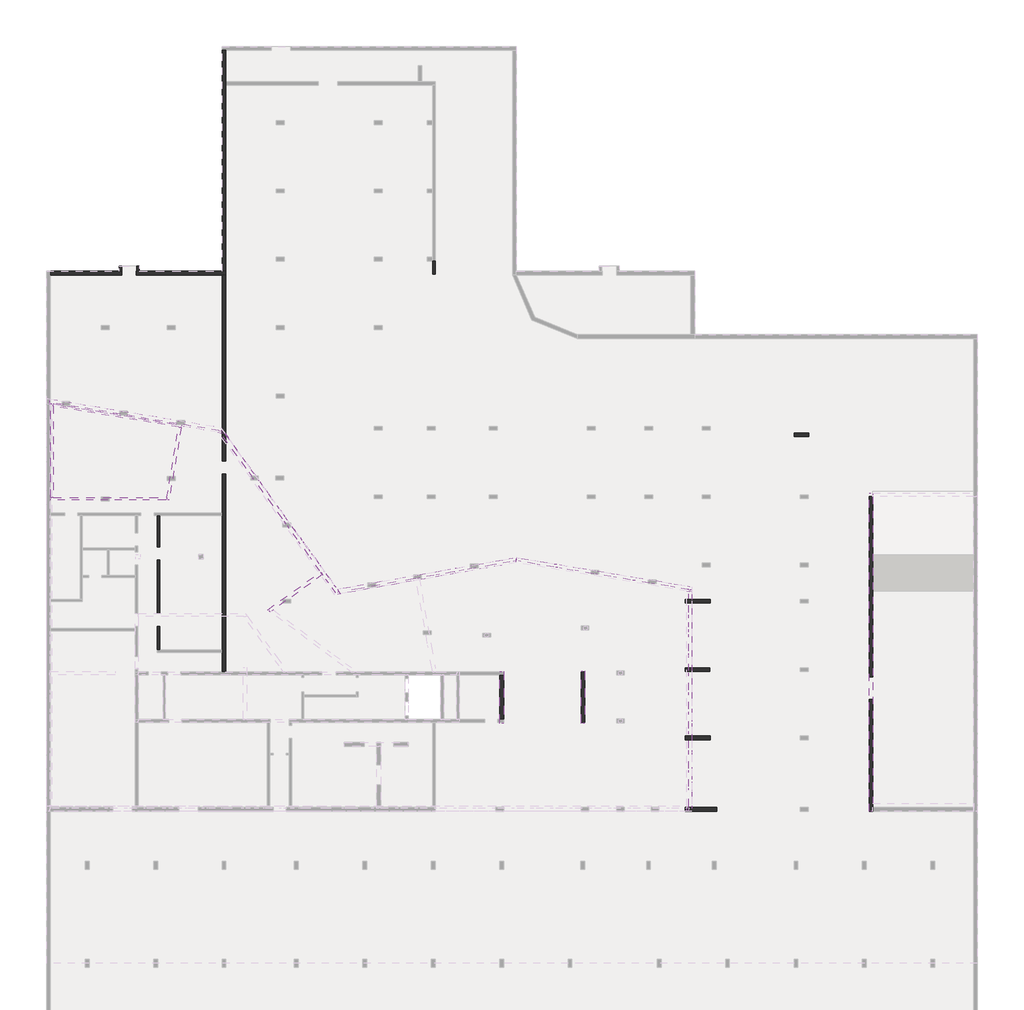
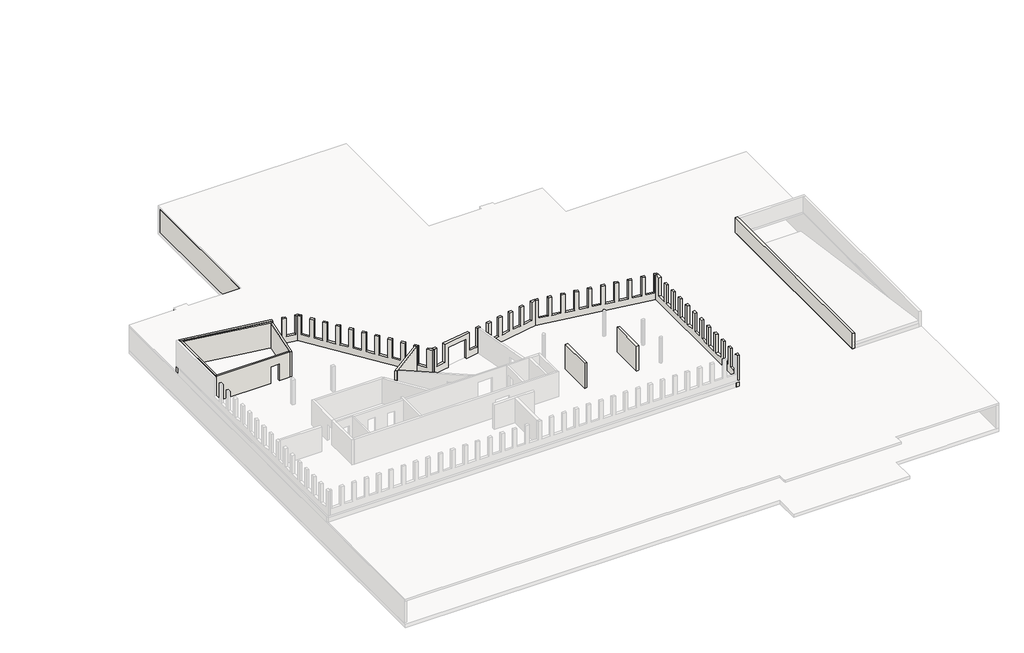
# One storey, part 3 of 4: 35 walls.
"""IFC4 building model written with IfcOpenShell, lengths in millimetres."""

from ifc_helpers import new_model, si_unit, point, frame, frame_2d, origin, place, context, project, spatial, polyline, circle_curve, trimmed, segment, composite_curve, outline, extrude, faceted_brep, element, save

model = new_model("IFC4")

# Units and contexts
model_context = context("Model", 3, world=origin())
ifc_project = project(units=[si_unit("LENGTHUNIT", "METRE", prefix="MILLI")], contexts=[model_context])

# Site, building, storey
site = spatial("IfcSite", under=ifc_project)
building = spatial("IfcBuilding", under=site)
storey = spatial("IfcBuildingStorey", under=building, Name="01_UG_OKFB_-4,20", Elevation=-4200.0)

# Walls
placement = place(None, origin())
element("IfcWall", 1, ObjectType="5dki Lochfassade 26cm C30/37", at=placement, inside=storey, context=model_context, shape_type="Brep", body=[
    faceted_brep([(13575.6085618, 29303.4331075, 3060.0), (13211.4553837, 29364.2425792, 3060.0), (12991.7792945, 29400.9260074, 3060.0), (12991.7792945, 29400.9260074, 710.0), (11926.5295409, 29578.8106961, 710.0), (11926.5295409, 29578.8106961, 3060.0), (11512.2657479, 29647.9880751, 3060.0), (11512.2657479, 29647.9880751, 710.0), (10447.0159943, 29825.8727639, 710.0), (10447.0159943, 29825.8727639, 3060.0), (130.0010047, 31548.6978518, 3060.0), (130.0010047, 31548.6978518, -150.0), (13211.4553837, 29364.2425792, -150.0), (13575.6085618, 29303.4331075, -150.0), (13034.6033862, 29657.3750221, 710.0), (13034.6033862, 29657.3750221, 3060.0), (13359.8955383, 29603.0549033, 3060.0), (13359.8955383, 29603.0549033, -150.0), (130.0010047, 31812.2980067, -150.0), (130.0010047, 31812.2980067, 3060.0), (10489.840086, 30082.3217786, 3060.0), (10489.840086, 30082.3217786, 710.0), (11555.0898396, 29904.4370898, 710.0), (11555.0898396, 29904.4370898, 3060.0), (11969.3536327, 29835.2597109, 3060.0), (11969.3536327, 29835.2597109, 710.0)], [[[0, 1, 2, 3, 4, 5, 6, 7, 8, 9, 10, 11, 12, 13]], [[14, 15, 16, 17, 18, 19, 20, 21, 22, 23, 24, 25]], [[13, 12, 11, 18, 17]], [[19, 10, 9, 20]], [[24, 23, 6, 5]], [[16, 15, 2, 1, 0]], [[11, 10, 19, 18]], [[0, 13, 17, 16]], [[8, 21, 20, 9]], [[22, 7, 6, 23]], [[21, 8, 7, 22]], [[5, 4, 25, 24]], [[3, 2, 15, 14]], [[4, 3, 14, 25]]]),
])
element("IfcWall", 2, ObjectType="5dki Lochfassade 26cm C30/37", at=placement, inside=storey, context=model_context, shape_type="Brep", body=[
    faceted_brep([(22268.004401, 16784.8468851, 3060.0), (21924.4906268, 17261.9817942, 3060.0), (21924.4906268, 17261.9817942, 710.0), (21293.4697845, 18138.4592307, 710.0), (21293.4697845, 18138.4592307, 3060.0), (21048.0727903, 18479.3115671, 3060.0), (21048.0727903, 18479.3115671, 710.0), (20417.0519481, 19355.7890035, 710.0), (20417.0519481, 19355.7890035, 3060.0), (20171.6549538, 19696.64134, 3060.0), (20171.6549538, 19696.64134, 710.0), (19540.6341116, 20573.1187764, 710.0), (19540.6341116, 20573.1187764, 3060.0), (19295.2371174, 20913.9711128, 3060.0), (19295.2371174, 20913.9711128, 710.0), (18664.2162751, 21790.4485493, 710.0), (18664.2162751, 21790.4485493, 3060.0), (18418.8192809, 22131.3008857, 3060.0), (18418.8192809, 22131.3008857, 710.0), (17787.7984387, 23007.7783222, 710.0), (17787.7984387, 23007.7783222, 3060.0), (17542.4014445, 23348.6306586, 3060.0), (17542.4014445, 23348.6306586, 710.0), (16911.3806022, 24225.1080951, 710.0), (16911.3806022, 24225.1080951, 3060.0), (16665.983608, 24565.9604315, 3060.0), (16665.983608, 24565.9604315, 710.0), (16034.9627658, 25442.4378679, 710.0), (16034.9627658, 25442.4378679, 3060.0), (15789.5657715, 25783.2902043, 3060.0), (15789.5657715, 25783.2902043, 710.0), (15158.5449293, 26659.7676408, 710.0), (15158.5449293, 26659.7676408, 3060.0), (14913.1479351, 27000.6199772, 3060.0), (14913.1479351, 27000.6199772, 710.0), (14282.1270928, 27877.0974137, 710.0), (14282.1270928, 27877.0974137, 3060.0), (14036.7300986, 28217.9497501, 3060.0), (14036.7300986, 28217.9497501, 710.0), (13405.7092564, 29094.4271866, 710.0), (13405.7092564, 29094.4271866, 3060.0), (13211.4553837, 29364.2425792, 3060.0), (13211.4553837, 29364.2425792, -150.0), (22268.004401, 16784.8468851, -150.0), (22135.4944541, 17413.8942192, 710.0), (22135.4944541, 17413.8942192, 3060.0), (22383.5041721, 17069.4128529, 3060.0), (22552.0750732, 16835.2706799, 3060.0), (22552.0750732, 16835.2706799, -150.0), (22383.5041721, 17069.4128529, -150.0), (13575.6085618, 29303.4331075, -150.0), (13575.6085618, 29303.4331075, 3060.0), (13616.7130837, 29246.3396115, 3060.0), (13616.7130837, 29246.3396115, 710.0), (14247.7339259, 28369.8621751, 710.0), (14247.7339259, 28369.8621751, 3060.0), (14493.1309201, 28029.0098387, 3060.0), (14493.1309201, 28029.0098387, 710.0), (15124.1517624, 27152.5324022, 710.0), (15124.1517624, 27152.5324022, 3060.0), (15369.5487566, 26811.6800658, 3060.0), (15369.5487566, 26811.6800658, 710.0), (16000.5695988, 25935.2026293, 710.0), (16000.5695988, 25935.2026293, 3060.0), (16245.966593, 25594.3502929, 3060.0), (16245.966593, 25594.3502929, 710.0), (16876.9874353, 24717.8728564, 710.0), (16876.9874353, 24717.8728564, 3060.0), (17122.3844295, 24377.02052, 3060.0), (17122.3844295, 24377.02052, 710.0), (17753.4052718, 23500.5430836, 710.0), (17753.4052718, 23500.5430836, 3060.0), (17998.802266, 23159.6907472, 3060.0), (17998.802266, 23159.6907472, 710.0), (18629.8231082, 22283.2133107, 710.0), (18629.8231082, 22283.2133107, 3060.0), (18875.2201024, 21942.3609743, 3060.0), (18875.2201024, 21942.3609743, 710.0), (19506.2409447, 21065.8835378, 710.0), (19506.2409447, 21065.8835378, 3060.0), (19751.6379389, 20725.0312014, 3060.0), (19751.6379389, 20725.0312014, 710.0), (20382.6587811, 19848.5537649, 710.0), (20382.6587811, 19848.5537649, 3060.0), (20628.0557754, 19507.7014285, 3060.0), (20628.0557754, 19507.7014285, 710.0), (21259.0766176, 18631.2239921, 710.0), (21259.0766176, 18631.2239921, 3060.0), (21504.4736118, 18290.3716557, 3060.0), (21504.4736118, 18290.3716557, 710.0)], [[[0, 1, 2, 3, 4, 5, 6, 7, 8, 9, 10, 11, 12, 13, 14, 15, 16, 17, 18, 19, 20, 21, 22, 23, 24, 25, 26, 27, 28, 29, 30, 31, 32, 33, 34, 35, 36, 37, 38, 39, 40, 41, 42, 43]], [[44, 45, 46, 47, 48, 49, 50, 51, 52, 53, 54, 55, 56, 57, 58, 59, 60, 61, 62, 63, 64, 65, 66, 67, 68, 69, 70, 71, 72, 73, 74, 75, 76, 77, 78, 79, 80, 81, 82, 83, 84, 85, 86, 87, 88, 89]], [[43, 42, 50, 49, 48]], [[51, 41, 40, 52]], [[56, 55, 37, 36]], [[60, 59, 33, 32]], [[64, 63, 29, 28]], [[68, 67, 25, 24]], [[72, 71, 21, 20]], [[76, 75, 17, 16]], [[80, 79, 13, 12]], [[84, 83, 9, 8]], [[88, 87, 5, 4]], [[47, 46, 45, 1, 0]], [[42, 41, 51, 50]], [[0, 43, 48, 47]], [[39, 53, 52, 40]], [[54, 38, 37, 55]], [[53, 39, 38, 54]], [[36, 35, 57, 56]], [[34, 33, 59, 58]], [[35, 34, 58, 57]], [[32, 31, 61, 60]], [[30, 29, 63, 62]], [[31, 30, 62, 61]], [[28, 27, 65, 64]], [[26, 25, 67, 66]], [[27, 26, 66, 65]], [[24, 23, 69, 68]], [[22, 21, 71, 70]], [[23, 22, 70, 69]], [[20, 19, 73, 72]], [[18, 17, 75, 74]], [[19, 18, 74, 73]], [[16, 15, 77, 76]], [[14, 13, 79, 78]], [[15, 14, 78, 77]], [[12, 11, 81, 80]], [[10, 9, 83, 82]], [[11, 10, 82, 81]], [[8, 7, 85, 84]], [[6, 5, 87, 86]], [[7, 6, 86, 85]], [[4, 3, 89, 88]], [[2, 1, 45, 44]], [[3, 2, 44, 89]]]),
])
element("IfcWall", 3, ObjectType="5dki Lochfassade 26cm C30/37", at=placement, inside=storey, context=model_context, shape_type="Brep", body=[
    faceted_brep([(34703.2430153, 18992.1564787, 710.0), (34703.2430153, 18992.1564787, 3060.0), (34289.7072944, 18918.7520679, 3060.0), (34289.7072944, 18918.7520679, 710.0), (33226.3297263, 18729.9978686, 710.0), (33226.3297263, 18729.9978686, 3060.0), (32812.7940054, 18656.5934577, 3060.0), (32812.7940054, 18656.5934577, 710.0), (31749.4164374, 18467.8392585, 710.0), (31749.4164374, 18467.8392585, 3060.0), (31335.8807164, 18394.4348476, 3060.0), (31335.8807164, 18394.4348476, 710.0), (30272.5031484, 18205.6806483, 710.0), (30272.5031484, 18205.6806483, 3060.0), (29858.9674275, 18132.2762375, 3060.0), (29858.9674275, 18132.2762375, 710.0), (28795.5898594, 17943.5220382, 710.0), (28795.5898594, 17943.5220382, 3060.0), (28731.5904499, 17932.1618613, 3060.0), (28485.4382351, 17888.4687596, 3060.0), (28382.0541385, 17870.1176274, 3060.0), (28382.0541385, 17870.1176274, 710.0), (27318.6765704, 17681.3634281, 710.0), (27318.6765704, 17681.3634281, 3060.0), (23971.0064488, 17087.1372452, 3060.0), (23971.0064488, 17087.1372452, 710.0), (22907.6288807, 16898.3830459, 710.0), (22907.6288807, 16898.3830459, 3060.0), (22552.0750732, 16835.2706799, 3060.0), (22552.0750732, 16835.2706799, -150.0), (24463.3121553, 17174.5236752, -150.0), (24463.3121553, 17174.5236752, 2410.0), (26924.8343036, 17611.454692, 2410.0), (26924.8343036, 17611.454692, -150.0), (28485.4382351, 17888.4687596, -150.0), (28731.5904499, 17932.1618613, -150.0), (36261.33607, 19268.7248546, -150.0), (36261.33607, 19268.7248546, 3060.0), (35766.6205834, 19180.910678, 3060.0), (35766.6205834, 19180.910678, 710.0), (34244.2664686, 19174.7503713, 3060.0), (34657.8021895, 19248.1547821, 3060.0), (34657.8021895, 19248.1547821, 710.0), (35721.1797576, 19436.9089814, 710.0), (35721.1797576, 19436.9089814, 3060.0), (36259.9888873, 19532.5499737, 3060.0), (36259.9888873, 19532.5499737, -150.0), (26879.3934778, 17867.4529955, -150.0), (26879.3934778, 17867.4529955, 2410.0), (24417.8713295, 17430.5219786, 2410.0), (24417.8713295, 17430.5219786, -150.0), (22383.5041721, 17069.4128529, -150.0), (22383.5041721, 17069.4128529, 3060.0), (22862.188055, 17154.3813493, 3060.0), (22862.188055, 17154.3813493, 710.0), (23925.565623, 17343.1355486, 710.0), (23925.565623, 17343.1355486, 3060.0), (27273.2357447, 17937.3617315, 3060.0), (27273.2357447, 17937.3617315, 710.0), (28336.6133127, 18126.1159308, 710.0), (28336.6133127, 18126.1159308, 3060.0), (28750.1490337, 18199.5203416, 3060.0), (28750.1490337, 18199.5203416, 710.0), (29813.5266017, 18388.2745409, 710.0), (29813.5266017, 18388.2745409, 3060.0), (30227.0623226, 18461.6789518, 3060.0), (30227.0623226, 18461.6789518, 710.0), (31290.4398907, 18650.433151, 710.0), (31290.4398907, 18650.433151, 3060.0), (31703.9756116, 18723.8375619, 3060.0), (31703.9756116, 18723.8375619, 710.0), (32767.3531797, 18912.5917612, 710.0), (32767.3531797, 18912.5917612, 3060.0), (33180.8889006, 18985.996172, 3060.0), (33180.8889006, 18985.996172, 710.0), (34244.2664686, 19174.7503713, 710.0)], [[[0, 1, 2, 3, 4, 5, 6, 7, 8, 9, 10, 11, 12, 13, 14, 15, 16, 17, 18, 19, 20, 21, 22, 23, 24, 25, 26, 27, 28, 29, 30, 31, 32, 33, 34, 35, 36, 37, 38, 39]], [[40, 41, 42, 43, 44, 45, 46, 47, 48, 49, 50, 51, 52, 53, 54, 55, 56, 57, 58, 59, 60, 61, 62, 63, 64, 65, 66, 67, 68, 69, 70, 71, 72, 73, 74, 75]], [[29, 51, 50, 30]], [[46, 36, 35, 34, 33, 47]], [[53, 52, 28, 27]], [[24, 23, 57, 56]], [[61, 60, 20, 19, 18, 17]], [[14, 13, 65, 64]], [[69, 68, 10, 9]], [[6, 5, 73, 72]], [[38, 37, 45, 44]], [[2, 1, 41, 40]], [[29, 28, 52, 51]], [[37, 36, 46, 45]], [[49, 31, 30, 50]], [[31, 49, 48, 32]], [[32, 48, 47, 33]], [[27, 26, 54, 53]], [[25, 24, 56, 55]], [[26, 25, 55, 54]], [[60, 59, 21, 20]], [[58, 57, 23, 22]], [[59, 58, 22, 21]], [[17, 16, 62, 61]], [[15, 14, 64, 63]], [[16, 15, 63, 62]], [[68, 67, 11, 10]], [[66, 65, 13, 12]], [[67, 66, 12, 11]], [[9, 8, 70, 69]], [[7, 6, 72, 71]], [[8, 7, 71, 70]], [[40, 75, 3, 2]], [[74, 73, 5, 4]], [[75, 74, 4, 3]], [[44, 43, 39, 38]], [[42, 41, 1, 0]], [[43, 42, 0, 39]]]),
])
element("IfcWall", 4, ObjectType="5dki Lochfassade 26cm C30/37", at=placement, inside=storey, context=model_context, shape_type="Brep", body=[
    faceted_brep([(49863.9990837, 16997.2336245, 3060.0), (49603.9990837, 17040.6506907, 3060.0), (49507.8677901, 17056.7035319, 3060.0), (49507.8677901, 17056.7035319, 710.0), (48442.6180365, 17234.5882205, 710.0), (48442.6180365, 17234.5882205, 3060.0), (48028.3542434, 17303.7655993, 3060.0), (48028.3542434, 17303.7655993, 710.0), (46963.1044898, 17481.6502878, 710.0), (46963.1044898, 17481.6502878, 3060.0), (46548.8406967, 17550.8276667, 3060.0), (46548.8406967, 17550.8276667, 710.0), (45483.5909431, 17728.7123552, 710.0), (45483.5909431, 17728.7123552, 3060.0), (45069.32715, 17797.8897341, 3060.0), (45069.32715, 17797.8897341, 710.0), (44004.0773964, 17975.7744226, 710.0), (44004.0773964, 17975.7744226, 3060.0), (43589.8136033, 18044.9518015, 3060.0), (43589.8136033, 18044.9518015, 710.0), (42524.5638497, 18222.83649, 710.0), (42524.5638497, 18222.83649, 3060.0), (42110.3000566, 18292.0138689, 3060.0), (42110.3000566, 18292.0138689, 710.0), (41045.050303, 18469.8985574, 710.0), (41045.050303, 18469.8985574, 3060.0), (40630.7865099, 18539.0759362, 3060.0), (40630.7865099, 18539.0759362, 710.0), (39565.5367563, 18716.9606248, 710.0), (39565.5367563, 18716.9606248, 3060.0), (39151.2729632, 18786.1380036, 3060.0), (39151.2729632, 18786.1380036, 710.0), (38086.0232096, 18964.0226921, 710.0), (38086.0232096, 18964.0226921, 3060.0), (37671.7594165, 19033.200071, 3060.0), (37671.7594165, 19033.200071, 710.0), (36606.5096629, 19211.0847595, 710.0), (36606.5096629, 19211.0847595, 3060.0), (36261.33607, 19268.7248546, 3060.0), (36261.33607, 19268.7248546, -150.0), (49603.9990837, 17040.6506907, -150.0), (49863.9990837, 16997.2336245, -150.0), (49550.6918818, 17313.1525467, 710.0), (49550.6918818, 17313.1525467, 3060.0), (49863.9990833, 17260.8337794, 3060.0), (49863.9990833, 17260.8337794, -150.0), (36259.9888873, 19532.5499737, -150.0), (36259.9888873, 19532.5499737, 3060.0), (36649.3337546, 19467.5337743, 3060.0), (36649.3337546, 19467.5337743, 710.0), (37714.5835082, 19289.6490858, 710.0), (37714.5835082, 19289.6490858, 3060.0), (38128.8473013, 19220.4717069, 3060.0), (38128.8473013, 19220.4717069, 710.0), (39194.0970549, 19042.5870184, 710.0), (39194.0970549, 19042.5870184, 3060.0), (39608.360848, 18973.4096395, 3060.0), (39608.360848, 18973.4096395, 710.0), (40673.6106016, 18795.524951, 710.0), (40673.6106016, 18795.524951, 3060.0), (41087.8743947, 18726.3475721, 3060.0), (41087.8743947, 18726.3475721, 710.0), (42153.1241483, 18548.4628836, 710.0), (42153.1241483, 18548.4628836, 3060.0), (42567.3879414, 18479.2855048, 3060.0), (42567.3879414, 18479.2855048, 710.0), (43632.637695, 18301.4008162, 710.0), (43632.637695, 18301.4008162, 3060.0), (44046.9014881, 18232.2234374, 3060.0), (44046.9014881, 18232.2234374, 710.0), (45112.1512417, 18054.3387489, 710.0), (45112.1512417, 18054.3387489, 3060.0), (45526.4150348, 17985.16137, 3060.0), (45526.4150348, 17985.16137, 710.0), (46591.6647884, 17807.2766815, 710.0), (46591.6647884, 17807.2766815, 3060.0), (47005.9285815, 17738.0993026, 3060.0), (47005.9285815, 17738.0993026, 710.0), (48071.1783351, 17560.2146141, 710.0), (48071.1783351, 17560.2146141, 3060.0), (48485.4421282, 17491.0372352, 3060.0), (48485.4421282, 17491.0372352, 710.0)], [[[0, 1, 2, 3, 4, 5, 6, 7, 8, 9, 10, 11, 12, 13, 14, 15, 16, 17, 18, 19, 20, 21, 22, 23, 24, 25, 26, 27, 28, 29, 30, 31, 32, 33, 34, 35, 36, 37, 38, 39, 40, 41]], [[42, 43, 44, 45, 46, 47, 48, 49, 50, 51, 52, 53, 54, 55, 56, 57, 58, 59, 60, 61, 62, 63, 64, 65, 66, 67, 68, 69, 70, 71, 72, 73, 74, 75, 76, 77, 78, 79, 80, 81]], [[41, 40, 39, 46, 45]], [[48, 47, 38, 37]], [[52, 51, 34, 33]], [[56, 55, 30, 29]], [[60, 59, 26, 25]], [[64, 63, 22, 21]], [[68, 67, 18, 17]], [[72, 71, 14, 13]], [[76, 75, 10, 9]], [[80, 79, 6, 5]], [[44, 43, 2, 1, 0]], [[39, 38, 47, 46]], [[0, 41, 45, 44]], [[37, 36, 49, 48]], [[35, 34, 51, 50]], [[36, 35, 50, 49]], [[33, 32, 53, 52]], [[31, 30, 55, 54]], [[32, 31, 54, 53]], [[29, 28, 57, 56]], [[27, 26, 59, 58]], [[28, 27, 58, 57]], [[25, 24, 61, 60]], [[23, 22, 63, 62]], [[24, 23, 62, 61]], [[21, 20, 65, 64]], [[19, 18, 67, 66]], [[20, 19, 66, 65]], [[17, 16, 69, 68]], [[15, 14, 71, 70]], [[16, 15, 70, 69]], [[13, 12, 73, 72]], [[11, 10, 75, 74]], [[12, 11, 74, 73]], [[9, 8, 77, 76]], [[7, 6, 79, 78]], [[8, 7, 78, 77]], [[5, 4, 81, 80]], [[3, 2, 43, 42]], [[4, 3, 42, 81]]]),
])
element("IfcWall", 5, ObjectType="5dki Lochfassade 26cm C30/37", at=placement, inside=storey, context=model_context, shape_type="Brep", body=[
    faceted_brep([(49603.9991105, -129.9989514, 3060.0), (49603.9991101, 130.0010486, 3060.0), (49603.9991099, 277.0124979, 3060.0), (49603.9991099, 277.0124979, 710.0), (49603.9991082, 1357.0124979, 710.0), (49603.9991082, 1357.0124979, 3060.0), (49603.9991075, 1777.0124979, 3060.0), (49603.9991075, 1777.0124979, 710.0), (49603.9991058, 2857.0124979, 710.0), (49603.9991058, 2857.0124979, 3060.0), (49603.9991052, 3277.0124979, 3060.0), (49603.9991052, 3277.0124979, 710.0), (49603.9991035, 4357.0124979, 710.0), (49603.9991035, 4357.0124979, 3060.0), (49603.9991028, 4777.0124979, 3060.0), (49603.9991028, 4777.0124979, 710.0), (49603.9991011, 5857.0124979, 710.0), (49603.9991011, 5857.0124979, 3060.0), (49603.9991005, 6277.0124979, 3060.0), (49603.9991005, 6277.0124979, 710.0), (49603.9990988, 7357.0124979, 710.0), (49603.9990988, 7357.0124979, 3060.0), (49603.9990981, 7777.0124979, 3060.0), (49603.9990981, 7777.0124979, 710.0), (49603.9990964, 8857.0124979, 710.0), (49603.9990964, 8857.0124979, 3060.0), (49603.9990958, 9277.0124979, 3060.0), (49603.9990958, 9277.0124979, 710.0), (49603.9990941, 10357.0124979, 710.0), (49603.9990941, 10357.0124979, 3060.0), (49603.9990934, 10777.0124979, 3060.0), (49603.9990934, 10777.0124979, 710.0), (49603.9990918, 11857.0124979, 710.0), (49603.9990918, 11857.0124979, 3060.0), (49603.9990911, 12277.0124979, 3060.0), (49603.9990911, 12277.0124979, 710.0), (49603.9990894, 13357.0124979, 710.0), (49603.9990894, 13357.0124979, 3060.0), (49603.9990888, 13777.0124979, 3060.0), (49603.9990888, 13777.0124979, 710.0), (49603.9990871, 14857.0124979, 710.0), (49603.9990871, 14857.0124979, 3060.0), (49603.9990864, 15277.0124979, 3060.0), (49603.9990864, 15277.0124979, 710.0), (49603.9990847, 16357.0124979, 710.0), (49603.9990847, 16357.0124979, 3060.0), (49603.9990837, 17040.6506907, 3060.0), (49603.9990837, 17040.6506907, -150.0), (49603.9991101, 130.0010486, -150.0), (49603.9991105, -129.9989514, -150.0), (49863.9991099, 277.0124983, 710.0), (49863.9991099, 277.0124983, 3060.0), (49863.9991105, -129.9989509, 3060.0), (49863.9991105, -129.9989509, -150.0), (49863.9990837, 16997.2336245, -150.0), (49863.9990837, 16997.2336245, 3060.0), (49863.9990847, 16357.0124983, 3060.0), (49863.9990847, 16357.0124983, 710.0), (49863.9990864, 15277.0124983, 710.0), (49863.9990864, 15277.0124983, 3060.0), (49863.9990871, 14857.0124983, 3060.0), (49863.9990871, 14857.0124983, 710.0), (49863.9990888, 13777.0124983, 710.0), (49863.9990888, 13777.0124983, 3060.0), (49863.9990894, 13357.0124983, 3060.0), (49863.9990894, 13357.0124983, 710.0), (49863.9990911, 12277.0124983, 710.0), (49863.9990911, 12277.0124983, 3060.0), (49863.9990918, 11857.0124983, 3060.0), (49863.9990918, 11857.0124983, 710.0), (49863.9990934, 10777.0124983, 710.0), (49863.9990934, 10777.0124983, 3060.0), (49863.9990941, 10357.0124983, 3060.0), (49863.9990941, 10357.0124983, 710.0), (49863.9990958, 9277.0124983, 710.0), (49863.9990958, 9277.0124983, 3060.0), (49863.9990964, 8857.0124983, 3060.0), (49863.9990964, 8857.0124983, 710.0), (49863.9990981, 7777.0124983, 710.0), (49863.9990981, 7777.0124983, 3060.0), (49863.9990988, 7357.0124983, 3060.0), (49863.9990988, 7357.0124983, 710.0), (49863.9991005, 6277.0124983, 710.0), (49863.9991005, 6277.0124983, 3060.0), (49863.9991011, 5857.0124983, 3060.0), (49863.9991011, 5857.0124983, 710.0), (49863.9991028, 4777.0124983, 710.0), (49863.9991028, 4777.0124983, 3060.0), (49863.9991035, 4357.0124983, 3060.0), (49863.9991035, 4357.0124983, 710.0), (49863.9991052, 3277.0124983, 710.0), (49863.9991052, 3277.0124983, 3060.0), (49863.9991058, 2857.0124983, 3060.0), (49863.9991058, 2857.0124983, 710.0), (49863.9991075, 1777.0124983, 710.0), (49863.9991075, 1777.0124983, 3060.0), (49863.9991082, 1357.0124983, 3060.0), (49863.9991082, 1357.0124983, 710.0)], [[[0, 1, 2, 3, 4, 5, 6, 7, 8, 9, 10, 11, 12, 13, 14, 15, 16, 17, 18, 19, 20, 21, 22, 23, 24, 25, 26, 27, 28, 29, 30, 31, 32, 33, 34, 35, 36, 37, 38, 39, 40, 41, 42, 43, 44, 45, 46, 47, 48, 49]], [[50, 51, 52, 53, 54, 55, 56, 57, 58, 59, 60, 61, 62, 63, 64, 65, 66, 67, 68, 69, 70, 71, 72, 73, 74, 75, 76, 77, 78, 79, 80, 81, 82, 83, 84, 85, 86, 87, 88, 89, 90, 91, 92, 93, 94, 95, 96, 97]], [[49, 48, 47, 54, 53]], [[55, 46, 45, 56]], [[42, 41, 60, 59]], [[38, 37, 64, 63]], [[34, 33, 68, 67]], [[30, 29, 72, 71]], [[26, 25, 76, 75]], [[22, 21, 80, 79]], [[18, 17, 84, 83]], [[14, 13, 88, 87]], [[10, 9, 92, 91]], [[96, 95, 6, 5]], [[52, 51, 2, 1, 0]], [[47, 46, 55, 54]], [[0, 49, 53, 52]], [[58, 43, 42, 59]], [[44, 57, 56, 45]], [[43, 58, 57, 44]], [[63, 62, 39, 38]], [[61, 60, 41, 40]], [[62, 61, 40, 39]], [[67, 66, 35, 34]], [[65, 64, 37, 36]], [[66, 65, 36, 35]], [[71, 70, 31, 30]], [[69, 68, 33, 32]], [[70, 69, 32, 31]], [[75, 74, 27, 26]], [[73, 72, 29, 28]], [[74, 73, 28, 27]], [[79, 78, 23, 22]], [[77, 76, 25, 24]], [[78, 77, 24, 23]], [[83, 82, 19, 18]], [[81, 80, 21, 20]], [[82, 81, 20, 19]], [[87, 86, 15, 14]], [[85, 84, 17, 16]], [[86, 85, 16, 15]], [[91, 90, 11, 10]], [[89, 88, 13, 12]], [[90, 89, 12, 11]], [[95, 94, 7, 6]], [[93, 92, 9, 8]], [[94, 93, 8, 7]], [[5, 4, 97, 96]], [[3, 2, 51, 50]], [[4, 3, 50, 97]]]),
])
element("IfcWall", 6, ObjectType="5dki STB-Wand Kern 30cm C30/37", at=placement, inside=storey, context=model_context, shape_type="SweptSolid", body=[
    extrude(outline(polyline([(34969.9993085, 6960.0016651), (34969.9993003, 10442.0123029), (35269.9993003, 10442.0122959), (35269.9993085, 6960.0016809), (34969.9993085, 6960.0016651)])), frame((0.0, 0.0, -4200.0), z_axis=(0.0, 0.0, 1.0), x_axis=(1.0, 0.0, 0.0)), (0.0, 0.0, 1.0), 3000.0),
])
element("IfcWall", 7, ObjectType="5dki STB-Wand 30cm WU C35/45", at=placement, inside=storey, context=model_context, shape_type="Brep", body=[
    faceted_brep([(13769.9996353, 41417.0011496, -1200.0), (13470.0000147, 41417.0011496, -1200.0), (169.9998112, 41417.0011496, -1200.0), (169.9998112, 41417.0011496, -4200.0), (5698.2798668, 41417.0011496, -4200.0), (5698.2798668, 41417.0011496, -2065.0), (6833.2798668, 41417.0011496, -2065.0), (6833.2798668, 41417.0011496, -4200.0), (13470.0000147, 41417.0011496, -4200.0), (13769.9996353, 41417.0011496, -4200.0), (169.9998112, 41717.0011496, -1200.0), (5491.9984219, 41717.0011496, -1200.0), (5691.9984219, 41717.0011496, -1200.0), (13469.9996419, 41717.0011496, -1200.0), (13769.9996419, 41717.0011496, -1200.0), (13769.9996419, 41717.0011496, -4200.0), (13469.9996419, 41717.0011496, -4200.0), (6833.2798668, 41717.0011496, -4200.0), (6833.2798668, 41717.0011496, -2065.0), (5698.2798668, 41717.0011496, -2065.0), (5698.2798668, 41717.0011496, -4200.0), (5691.9984219, 41717.0011496, -4200.0), (5491.9984219, 41717.0011496, -4200.0), (169.9998112, 41717.0011496, -4200.0)], [[[0, 1, 2, 3, 4, 5, 6, 7, 8, 9]], [[10, 11, 12, 13, 14, 15, 16, 17, 18, 19, 20, 21, 22, 23]], [[3, 23, 22, 21, 20, 4]], [[15, 9, 8, 7, 17, 16]], [[2, 1, 0, 14, 13, 12, 11, 10]], [[3, 2, 10, 23]], [[0, 9, 15, 14]], [[6, 18, 17, 7]], [[18, 6, 5, 19]], [[19, 5, 4, 20]]]),
])
element("IfcWall", 8, ObjectType="5dki STB-Wand 30cm WU C35/45", at=placement, inside=storey, context=model_context, shape_type="Brep", body=[
    faceted_brep([(13769.9996419, 41717.0011496, -4200.0), (13769.9999561, 56135.574851, -4200.0), (13769.9999615, 56385.574851, -4200.0), (13770.0000147, 58825.9289901, -4200.0), (13770.0000147, 58825.9289901, -1200.0), (13769.9999615, 56385.574851, -1200.0), (13769.9999561, 56135.574851, -1200.0), (13769.9996419, 41717.0011496, -1200.0), (13469.9996419, 41717.0011496, -4200.0), (13469.9996419, 41717.0011496, -1200.0), (13470.0000147, 58825.9289986, -1200.0), (13470.0000147, 58825.9289986, -4200.0)], [[[0, 1, 2, 3, 4, 5, 6, 7]], [[8, 9, 10, 11]], [[3, 2, 1, 0, 8, 11]], [[7, 6, 5, 4, 10, 9]], [[4, 3, 11, 10]], [[0, 7, 9, 8]]]),
])
element("IfcWall", 9, ObjectType="5dki STB-Wand 20cm WU C30/37", at=placement, inside=storey, context=model_context, shape_type="SweptSolid", body=[
    extrude(outline(polyline([(5691.9984311, 42095.9291846), (5691.9984219, 41717.0011496), (5491.9984219, 41717.0011496), (5491.9984311, 42095.9291895), (5691.9984311, 42095.9291846)])), frame((0.0, 0.0, -4200.0), z_axis=(0.0, 0.0, 1.0), x_axis=(1.0, 0.0, 0.0)), (0.0, 0.0, 1.0), 3000.0),
])
element("IfcWall", 10, ObjectType="5dki STB-Wand 20cm WU C30/37", at=placement, inside=storey, context=model_context, shape_type="SweptSolid", body=[
    extrude(outline(polyline([(6842.0004993, 41717.0011496), (6842.0004993, 42095.9291528), (7042.0004993, 42095.9291528), (7042.0004993, 41717.0011496), (6842.0004993, 41717.0011496)])), frame((0.0, 0.0, -4200.0), z_axis=(0.0, 0.0, 1.0), x_axis=(1.0, 0.0, 0.0)), (0.0, 0.0, 1.0), 3000.0),
])
element("IfcWall", 11, ObjectType="5dki Überzug 40cm C30/37", at=placement, inside=storey, context=model_context, shape_type="Brep", body=[
    faceted_brep([(-130.0001888, 31450.1765724, -950.0), (13131.5260697, 29235.6513279, -950.0), (13691.7617284, 29142.0982945, -950.0), (13691.7617284, 29142.0982945, -400.0), (13131.5260697, 29235.6513279, -400.0), (269.9998112, 31383.3810859, -400.0), (-130.0001888, 31450.1765724, -400.0), (-130.0001888, 31855.7152722, -950.0), (-130.0001888, 31855.7152722, -400.0), (13359.8955383, 29603.0549033, -400.0), (13359.8955383, 29603.0549033, -950.0)], [[[0, 1, 2, 3, 4, 5, 6]], [[7, 8, 9, 10]], [[2, 1, 0, 7, 10]], [[6, 5, 4, 3, 9, 8]], [[3, 2, 10, 9]], [[0, 6, 8, 7]]]),
])
element("IfcWall", 12, ObjectType="5dki Überzug 40cm C30/37", at=placement, inside=storey, context=model_context, shape_type="Brep", body=[
    faceted_brep([(13131.5260697, 29235.6513279, -950.0), (22205.8122165, 16631.6190563, -950.0), (22205.8122165, 16631.6190563, -400.0), (13131.5260697, 29235.6513279, -400.0), (13691.7617284, 29142.0982945, -950.0), (13691.7617284, 29142.0982945, -400.0), (22383.5041721, 17069.4128529, -400.0), (22642.8440199, 16709.1941252, -400.0), (22642.8440199, 16709.1941252, -950.0), (22383.5041721, 17069.4128529, -950.0)], [[[0, 1, 2, 3]], [[4, 5, 6, 7, 8, 9]], [[1, 0, 4, 9, 8]], [[3, 2, 7, 6, 5]], [[0, 3, 5, 4]], [[2, 1, 8, 7]]]),
])
element("IfcWall", 13, ObjectType="5dki Überzug 40cm C30/37", at=placement, inside=storey, context=model_context, shape_type="SweptSolid", body=[
    extrude(outline(polyline([(36262.0614761, 19126.665175), (22642.8440199, 16709.1941252), (22383.5041721, 17069.4128529), (36259.9888873, 19532.5499737), (36262.0614761, 19126.665175)])), frame((0.0, 0.0, -950.0), z_axis=(0.0, 0.0, 1.0), x_axis=(1.0, 0.0, 0.0)), (0.0, 0.0, 1.0), 550.0),
])
element("IfcWall", 14, ObjectType="5dki Überzug 40cm C30/37", at=placement, inside=storey, context=model_context, shape_type="Brep", body=[
    faceted_brep([(36262.0614761, 19126.665175, -950.0), (49463.9990838, 16922.090566, -950.0), (49863.9990839, 16855.2950796, -950.0), (49863.9990839, 16855.2950796, -400.0), (49463.9990838, 16922.090566, -400.0), (36262.0614761, 19126.665175, -400.0), (36259.9888873, 19532.5499737, -950.0), (36259.9888873, 19532.5499737, -400.0), (49863.9990833, 17260.8337794, -400.0), (49863.9990833, 17260.8337794, -950.0)], [[[0, 1, 2, 3, 4, 5]], [[6, 7, 8, 9]], [[2, 1, 0, 6, 9]], [[5, 4, 3, 8, 7]], [[0, 5, 7, 6]], [[3, 2, 9, 8]]]),
])
element("IfcWall", 15, ObjectType="5dki Überzug 40cm C30/37", at=placement, inside=storey, context=model_context, shape_type="Brep", body=[
    faceted_brep([(49463.9990838, 16922.090566, -950.0), (49463.9991099, 270.0010491, -950.0), (49463.9991105, -129.9989509, -950.0), (49463.9991105, -129.9989509, -400.0), (49463.9991099, 270.0010491, -400.0), (49463.9990838, 16922.090566, -400.0), (49863.9990839, 16855.2950796, -950.0), (49863.9990839, 16855.2950796, -400.0), (49863.9991105, -129.9989509, -400.0), (49863.9991105, -129.9989509, -950.0)], [[[0, 1, 2, 3, 4, 5]], [[6, 7, 8, 9]], [[2, 1, 0, 6, 9]], [[5, 4, 3, 8, 7]], [[0, 5, 7, 6]], [[3, 2, 9, 8]]]),
])
element("IfcWall", 16, ObjectType="5dki STB-Wand 20cm C25/30", at=placement, inside=storey, context=model_context, shape_type="Brep", body=[
    faceted_brep([(8640.0002224, 22769.9812381, -1200.0), (8640.0000033, 12367.0009111, -1200.0), (8640.0000033, 12367.0009111, -4200.0), (8640.0000412, 14168.6536032, -4200.0), (8640.0000412, 14168.6536032, -2065.0), (8640.0000625, 15178.6536032, -2065.0), (8640.0000625, 15178.6536032, -4200.0), (8640.0001503, 19346.7665193, -4200.0), (8640.0001503, 19346.7665193, -2065.0), (8640.0001715, 20356.7665193, -2065.0), (8640.0001715, 20356.7665193, -4200.0), (8640.0002224, 22769.9812381, -4200.0), (8440.0000033, 12367.0009111, -1200.0), (8440.0002224, 22769.9812432, -1200.0), (8440.0002224, 22769.9812432, -4200.0), (8440.0001715, 20356.7665235, -4200.0), (8440.0001715, 20356.7665235, -2065.0), (8440.0001503, 19346.7665235, -2065.0), (8440.0001503, 19346.7665235, -4200.0), (8440.0000625, 15178.6536074, -4200.0), (8440.0000625, 15178.6536074, -2065.0), (8440.0000412, 14168.6536074, -2065.0), (8440.0000412, 14168.6536074, -4200.0), (8440.0000033, 12367.0009111, -4200.0)], [[[0, 1, 2, 3, 4, 5, 6, 7, 8, 9, 10, 11]], [[12, 13, 14, 15, 16, 17, 18, 19, 20, 21, 22, 23]], [[2, 23, 22, 3]], [[14, 11, 10, 15]], [[18, 7, 6, 19]], [[1, 0, 13, 12]], [[2, 1, 12, 23]], [[0, 11, 14, 13]], [[17, 8, 7, 18]], [[8, 17, 16, 9]], [[9, 16, 15, 10]], [[21, 4, 3, 22]], [[4, 21, 20, 5]], [[5, 20, 19, 6]]]),
])
element("IfcWall", 17, ObjectType="5dki STB-Wand 20cm C25/30", at=placement, inside=storey, context=model_context, shape_type="SweptSolid", body=[
    extrude(outline(composite_curve([segment(polyline([(29770.0264985, 41485.574441), (29970.0264985, 41485.5744362)]), True, "CONTINUOUS"), segment(trimmed(circle_curve(frame_2d((24970.0264985, 41485.574557)), 5000.0), [point((29970.0264985, 41485.5744362))], [point((28014.6541125, 37519.4375584))], False, "CARTESIAN"), True, "CONTINUOUS"), segment(polyline([(28014.6541125, 37519.4375584), (27892.8690079, 37678.0830383)]), True, "CONTINUOUS"), segment(trimmed(circle_curve(frame_2d((24970.0264985, 41485.574557)), 4800.0), [point((27892.8690079, 37678.0830383))], [point((29770.0264985, 41485.574441))], True, "CARTESIAN"), True, "CONTINUOUS")], self_intersect=False)), frame((0.0, 0.0, -4200.0), z_axis=(0.0, 0.0, 1.0), x_axis=(1.0, 0.0, 0.0)), (0.0, 0.0, 1.0), 3000.0),
])
element("IfcWall", 18, ObjectType="5dki STB-Wand 20cm C25/30", at=placement, inside=storey, context=model_context, shape_type="SweptSolid", body=[
    extrude(outline(polyline([(29970.0264985, 42485.5744872), (29970.0264985, 41485.5744386), (29770.0264985, 41485.5744386), (29770.0264985, 42485.5744872), (29970.0264985, 42485.5744872)])), frame((0.0, 0.0, -4200.0), z_axis=(0.0, 0.0, 1.0), x_axis=(1.0, 0.0, 0.0)), (0.0, 0.0, 1.0), 3000.0),
])
element("IfcWall", 19, ObjectType="5dki STB-Wand 20cm C30/37", at=placement, inside=storey, context=model_context, shape_type="Brep", body=[
    faceted_brep([(179.9999842, 24166.8495132, 3060.0), (379.9999842, 24166.8495132, 3060.0), (9187.7304791, 24166.8495132, 3060.0), (9187.7304791, 24166.8495132, -150.0), (7830.000204, 24166.8495132, -150.0), (7830.000204, 24166.8495132, 1985.0), (6820.000204, 24166.8495132, 1985.0), (6820.000204, 24166.8495132, -150.0), (379.9999842, 24166.8495132, -150.0), (179.9999842, 24166.8495132, -150.0), (9154.332736, 23966.8495132, 3060.0), (179.9999842, 23966.8495132, 3060.0), (179.9999842, 23966.8495132, -150.0), (6820.000204, 23966.8495132, -150.0), (6820.000204, 23966.8495132, 1985.0), (7830.000204, 23966.8495132, 1985.0), (7830.000204, 23966.8495132, -150.0), (9154.332736, 23966.8495132, -150.0)], [[[0, 1, 2, 3, 4, 5, 6, 7, 8, 9]], [[10, 11, 12, 13, 14, 15, 16, 17]], [[12, 9, 8, 7, 13]], [[3, 17, 16, 4]], [[2, 1, 0, 11, 10]], [[0, 9, 12, 11]], [[3, 2, 10, 17]], [[15, 5, 4, 16]], [[5, 15, 14, 6]], [[6, 14, 13, 7]]]),
])
element("IfcWall", 20, ObjectType="5dki STB-Wand 20cm C30/37", at=placement, inside=storey, context=model_context, shape_type="Brep", body=[
    faceted_brep([(379.9999842, 24166.8495132, -150.0), (379.9999842, 31253.489127, -150.0), (379.9999842, 31456.2584769, -150.0), (379.9999842, 31456.2584769, 3060.0), (379.9999842, 31253.489127, 3060.0), (379.9999842, 24166.8495132, 3060.0), (179.9999842, 24166.8495132, -150.0), (179.9999842, 24166.8495132, 3060.0), (179.9999842, 31489.6562201, 3060.0), (179.9999842, 31489.6562201, -150.0)], [[[0, 1, 2, 3, 4, 5]], [[6, 7, 8, 9]], [[2, 1, 0, 6, 9]], [[5, 4, 3, 8, 7]], [[0, 5, 7, 6]], [[3, 2, 9, 8]]]),
])
element("IfcWall", 21, ObjectType="5dki STB-Wand 20cm C30/37", at=placement, inside=storey, context=model_context, shape_type="Brep", body=[
    faceted_brep([(379.9999842, 31253.489127, -150.0), (10100.0728462, 29630.3466386, -150.0), (10297.3413191, 29597.4050296, -150.0), (10297.3413191, 29597.4050296, 3060.0), (10100.0728462, 29630.3466386, 3060.0), (379.9999842, 31253.489127, 3060.0), (379.9999842, 31456.2584769, -150.0), (379.9999842, 31456.2584769, 3060.0), (10330.282928, 29794.6735025, 3060.0), (10330.282928, 29794.6735025, -150.0)], [[[0, 1, 2, 3, 4, 5]], [[6, 7, 8, 9]], [[2, 1, 0, 6, 9]], [[5, 4, 3, 8, 7]], [[0, 5, 7, 6]], [[3, 2, 9, 8]]]),
])
element("IfcWall", 22, ObjectType="5dki STB-Wand 20cm C30/37", at=placement, inside=storey, context=model_context, shape_type="Brep", body=[
    faceted_brep([(10100.0728462, 29630.3466386, -150.0), (9187.7304791, 24166.8495132, -150.0), (9154.332736, 23966.8495132, -150.0), (9154.332736, 23966.8495132, 3060.0), (9187.7304791, 24166.8495132, 3060.0), (10100.0728462, 29630.3466386, 3060.0), (10297.3413191, 29597.4050296, -150.0), (10297.3413191, 29597.4050296, 3060.0), (9357.1020859, 23966.8495132, 3060.0), (9357.1020859, 23966.8495132, -150.0)], [[[0, 1, 2, 3, 4, 5]], [[6, 7, 8, 9]], [[2, 1, 0, 6, 9]], [[5, 4, 3, 8, 7]], [[0, 5, 7, 6]], [[3, 2, 9, 8]]]),
])
element("IfcWall", 23, ObjectType="5dki STB-Wand 25cm C30/37", at=placement, inside=storey, context=model_context, shape_type="Brep", body=[
    faceted_brep([(21084.845921, 18397.4352698, -150.0), (16996.4717259, 15463.7807738, -150.0), (16996.4717259, 15463.7807738, 3060.0), (21084.845921, 18397.4352698, 3060.0), (21230.5955347, 18194.3169542, -150.0), (21230.5955347, 18194.3169542, 3060.0), (17421.0951098, 15460.7711691, 3060.0), (17207.6873918, 15307.63829, 3060.0), (17207.6873918, 15307.63829, -150.0), (17421.0951098, 15460.7711691, -150.0)], [[[0, 1, 2, 3]], [[4, 5, 6, 7, 8, 9]], [[1, 0, 4, 9, 8]], [[3, 2, 7, 6, 5]], [[0, 3, 5, 4]], [[2, 1, 8, 7]]]),
])
element("IfcWall", 24, ObjectType="5dki STB-Wand 30cm C30/37", at=placement, inside=storey, context=model_context, shape_type="SweptSolid", body=[
    extrude(outline(polyline([(34969.9990839, 6680.0000532), (34969.9990776, 10702.0125181), (35269.9990776, 10702.0125186), (35269.9990839, 6680.0000537), (34969.9990839, 6680.0000532)])), frame((0.0, 0.0, -150.0), z_axis=(0.0, 0.0, 1.0), x_axis=(1.0, 0.0, 0.0)), (0.0, 0.0, 1.0), 3210.0),
])
element("IfcWall", 25, ObjectType="5dki STB-Wand 30cm C30/37", at=placement, inside=storey, context=model_context, shape_type="SweptSolid", body=[
    extrude(outline(polyline([(41269.9990703, 6680.000074), (41269.9990703, 10722.0122605), (41569.9990703, 10722.0122605), (41569.9990703, 6680.000074), (41269.9990703, 6680.000074)])), frame((0.0, 0.0, -150.0), z_axis=(0.0, 0.0, 1.0), x_axis=(1.0, 0.0, 0.0)), (0.0, 0.0, 1.0), 3210.0),
])
element("IfcWall", 26, ObjectType="5dki STB-Wand 30cm C30/37", at=placement, inside=storey, context=model_context, shape_type="SweptSolid", body=[
    extrude(outline(polyline([(51769.9990338, -130.0011115), (49359.7433415, -130.0010492), (49359.7433493, 169.9989508), (51769.9990416, 169.9988885), (51769.9990338, -130.0011115)])), frame((0.0, 0.0, -4200.0), z_axis=(0.0, 0.0, 1.0), x_axis=(1.0, 0.0, 0.0)), (0.0, 0.0, 1.0), 3000.0),
])
element("IfcWall", 27, ObjectType="5dki STB-Wand 30cm C30/37", at=placement, inside=storey, context=model_context, shape_type="SweptSolid", body=[
    extrude(outline(polyline([(51269.9991678, 5385.5739763), (49359.7434752, 5385.5740223), (49359.7434824, 5685.5740223), (51269.999175, 5685.5739763), (51269.9991678, 5385.5739763)])), frame((0.0, 0.0, -4200.0), z_axis=(0.0, 0.0, 1.0), x_axis=(1.0, 0.0, 0.0)), (0.0, 0.0, 1.0), 3000.0),
])
element("IfcWall", 28, ObjectType="5dki STB-Wand 30cm C30/37", at=placement, inside=storey, context=model_context, shape_type="SweptSolid", body=[
    extrude(outline(polyline([(51259.7436118, 10685.5739759), (49359.7436118, 10685.5739759), (49359.7436118, 10985.5739759), (51259.7436118, 10985.5739759), (51259.7436118, 10685.5739759)])), frame((0.0, 0.0, -4200.0), z_axis=(0.0, 0.0, 1.0), x_axis=(1.0, 0.0, 0.0)), (0.0, 0.0, 1.0), 3000.0),
])
element("IfcWall", 29, ObjectType="5dki STB-Wand 30cm C30/37", at=placement, inside=storey, context=model_context, shape_type="SweptSolid", body=[
    extrude(outline(polyline([(51269.9994313, 15985.5739746), (49359.7437402, 15985.5739746), (49359.7437402, 16285.5739746), (51269.9994313, 16285.5739746), (51269.9994313, 15985.5739746)])), frame((0.0, 0.0, -4200.0), z_axis=(0.0, 0.0, 1.0), x_axis=(1.0, 0.0, 0.0)), (0.0, 0.0, 1.0), 3000.0),
])
element("IfcWall", 30, ObjectType="5dki STB-Wand 30cm C30/37", at=placement, inside=storey, context=model_context, shape_type="SweptSolid", body=[
    extrude(outline(polyline([(41269.9993207, 6740.0003794), (41269.9993207, 10662.0127967), (41569.9993207, 10662.0127967), (41569.9993207, 6740.0003794), (41269.9993207, 6740.0003794)])), frame((0.0, 0.0, -4200.0), z_axis=(0.0, 0.0, 1.0), x_axis=(1.0, 0.0, 0.0)), (0.0, 0.0, 1.0), 3000.0),
])
element("IfcWall", 31, ObjectType="5dki STB-Wand 30cm C30/37", at=placement, inside=storey, context=model_context, shape_type="Brep", body=[
    faceted_brep([(13469.9992195, 10662.0127998, -1200.0), (13469.9992584, 12167.0009111, -1200.0), (13469.9992636, 12367.0009111, -1200.0), (13469.9995325, 22769.9811151, -1200.0), (13469.9995377, 22969.9811151, -1200.0), (13470.0000147, 41417.0011496, -1200.0), (13470.0000147, 41417.0011496, -4200.0), (13469.9996417, 26991.6497937, -4200.0), (13469.9996417, 26991.6497937, -2065.0), (13469.9996156, 25981.6497937, -2065.0), (13469.9996156, 25981.6497937, -4200.0), (13469.9995377, 22969.9811151, -4200.0), (13469.9995325, 22769.9811151, -4200.0), (13469.9992636, 12367.0009111, -4200.0), (13469.9992584, 12167.0009111, -4200.0), (13469.9992195, 10662.0127998, -4200.0), (13770.0000147, 41417.0011496, -1200.0), (13769.9992195, 10662.0127928, -1200.0), (13769.9992195, 10662.0127928, -4200.0), (13769.9996156, 25981.6497859, -4200.0), (13769.9996156, 25981.6497859, -2065.0), (13769.9996417, 26991.6497859, -2065.0), (13769.9996417, 26991.6497859, -4200.0), (13770.0000147, 41417.0011496, -4200.0)], [[[0, 1, 2, 3, 4, 5, 6, 7, 8, 9, 10, 11, 12, 13, 14, 15]], [[16, 17, 18, 19, 20, 21, 22, 23]], [[18, 15, 14, 13, 12, 11, 10, 19]], [[6, 23, 22, 7]], [[5, 4, 3, 2, 1, 0, 17, 16]], [[0, 15, 18, 17]], [[6, 5, 16, 23]], [[9, 20, 19, 10]], [[20, 9, 8, 21]], [[21, 8, 7, 22]]]),
])
element("IfcWall", 32, ObjectType="5dki STB-Wand 30cm C30/37", at=placement, inside=storey, context=model_context, shape_type="Brep", body=[
    faceted_brep([(63879.9990521, 24235.5733256, -4200.0), (63879.9990521, 24235.5733256, -950.0), (63879.9990521, -130.0014231, -950.0), (63879.9990521, -130.0014231, -4200.0), (63879.9990521, 8525.5736736, -4200.0), (63879.9990521, 8525.5736736, -1940.0), (63879.9990521, 10285.5736736, -1940.0), (63879.9990521, 10285.5736736, -4200.0), (63579.9990521, 24235.5733256, -950.0), (63579.9990521, 24235.5733256, -4200.0), (63579.9990521, 10285.5736736, -4200.0), (63579.9990521, 10285.5736736, -1940.0), (63579.9990521, 8525.5736736, -1940.0), (63579.9990521, 8525.5736736, -4200.0), (63579.9990521, -130.0014153, -4200.0), (63579.9990521, -130.0014153, -950.0)], [[[0, 1, 2, 3, 4, 5, 6, 7]], [[8, 9, 10, 11, 12, 13, 14, 15]], [[9, 0, 7, 10]], [[3, 14, 13, 4]], [[1, 0, 9, 8]], [[2, 1, 8, 15]], [[12, 5, 4, 13]], [[5, 12, 11, 6]], [[6, 11, 10, 7]], [[3, 2, 15, 14]]]),
])
element("IfcWall", 33, ObjectType="5dki STB-Wand 30cm C30/37", at=placement, inside=storey, context=model_context, shape_type="SweptSolid", body=[
    extrude(outline(polyline([(58900.9911095, 28885.5737407), (57769.9997489, 28885.5737407), (57769.9997489, 29185.5737407), (58901.6780246, 29185.5737407), (58900.9911095, 28885.5737407)])), frame((0.0, 0.0, -4200.0), z_axis=(0.0, 0.0, 1.0), x_axis=(1.0, 0.0, 0.0)), (0.0, 0.0, 1.0), 3000.0),
])
element("IfcWall", 34, ObjectType="5dki STB-Wand 30cm C30/37", at=placement, inside=storey, context=model_context, shape_type="Brep", body=[
    faceted_brep([(63880.0003229, -132.4012776, -950.0), (63880.0003229, 24235.5733256, -950.0), (63880.0003229, 24535.5733256, -950.0), (63880.0003229, 24535.5733256, 1000.0), (63880.0003229, 24235.5733256, 1000.0), (63880.0003229, -132.4012776, 1000.0), (63580.0003229, -132.4012776, -950.0), (63580.0003229, -132.4012776, 1000.0), (63580.0003229, 24535.5733256, 1000.0), (63580.0003229, 24535.5733256, -950.0)], [[[0, 1, 2, 3, 4, 5]], [[6, 7, 8, 9]], [[2, 1, 0, 6, 9]], [[5, 4, 3, 8, 7]], [[0, 5, 7, 6]], [[3, 2, 9, 8]]]),
])
element("IfcWall", 35, ObjectType="5dki STB-Wand 30cm C30/37", at=placement, inside=storey, context=model_context, shape_type="SweptSolid", body=[
    extrude(outline(composite_curve([segment(polyline([(58900.9911095, 28885.5737407), (58901.6780246, 29185.5737407)]), True, "CONTINUOUS"), segment(trimmed(circle_curve(frame_2d((58879.1244608, 24184.4722642)), 5001.1523313), [point((58901.6780246, 29185.5737407))], [point((63879.9813284, 24238.834296))], False, "CARTESIAN"), True, "CONTINUOUS"), segment(polyline([(63879.9813284, 24238.834296), (63579.9990521, 24235.5733256)]), True, "CONTINUOUS"), segment(trimmed(circle_curve(frame_2d((58879.1244608, 24184.4722642)), 4701.1523313), [point((63579.9990521, 24235.5733256))], [point((58900.9911095, 28885.5737407))], True, "CARTESIAN"), True, "CONTINUOUS")], self_intersect=False)), frame((0.0, 0.0, -4200.0), z_axis=(0.0, 0.0, 1.0), x_axis=(1.0, 0.0, 0.0)), (0.0, 0.0, 1.0), 3000.0),
])

save(model, "model.ifc")

# Revit data of these elements
# Type "5dki Lochfassade 26cm C30/37"
#   Type Comments = ""
#   Description = ""
#   cpiComponentType = "Wall"
#   cpiFitMatchKey = "5D-KI-STB-OB-W-LF"
#   5d Materialgüte = "C35/45"
#   Filter Tragend / Nichttragend = yes
#   5dki WU = no
#   Layers, outside or top first: 0.260 m "5d Beton - Stahlbeton" (function 1)
# Type "5dki STB-Wand Kern 30cm C30/37"
#   Type Comments = ""
#   Description = ""
#   cpiComponentType = "Wall"
#   cpiFitMatchKey = "5D-KI-STB-OB-W-K"
#   5d Materialgüte = "C30/37"
#   Filter Tragend / Nichttragend = yes
#   5dki WU = no
#   Layers, outside or top first: 0.300 m "5d Beton - Stahlbeton" (function 1)
# Type "5dki STB-Wand 30cm WU C35/45"
#   Type Comments = ""
#   Description = ""
#   cpiComponentType = "Wall"
#   cpiFitMatchKey = "5D-KI-STB-OB-W"
#   5d Materialgüte = "C35/45"
#   Filter Tragend / Nichttragend = yes
#   5dki WU = yes
#   Layers, outside or top first: 0.300 m "5d Beton - Stahlbeton WU" (function 1)
# Type "5dki STB-Wand 20cm WU C30/37"
#   Type Comments = ""
#   Description = ""
#   cpiComponentType = "Wall"
#   cpiFitMatchKey = "5D-KI-STB-OB-W"
#   5d Materialgüte = "C30/37"
#   Filter Tragend / Nichttragend = yes
#   5dki WU = yes
#   Layers, outside or top first: 0.200 m "5d Beton - Stahlbeton WU" (function 1)
# Type "5dki Überzug 40cm C30/37"
#   Type Comments = ""
#   Description = ""
#   cpiComponentType = "Beam"
#   cpiFitMatchKey = "5D-KI-STB-OB-TR-UEZ"
#   5d Materialgüte = "C30/37"
#   Filter Tragend / Nichttragend = yes
#   Layers, outside or top first: 0.400 m "5d Beton - Stahlbeton" (function 1)
# Type "5dki STB-Wand 20cm C25/30"
#   Type Comments = ""
#   Description = ""
#   cpiComponentType = "Wall"
#   cpiFitMatchKey = "5D-KI-STB-OB-W"
#   5d Materialgüte = "C25/30"
#   Filter Tragend / Nichttragend = yes
#   5dki WU = no
#   Layers, outside or top first: 0.200 m "5d Beton - Stahlbeton" (function 1)
# Type "5dki STB-Wand 20cm C30/37"
#   Type Comments = ""
#   Description = ""
#   cpiComponentType = "Wall"
#   cpiFitMatchKey = "5D-KI-STB-OB-W"
#   5d Materialgüte = "C30/37"
#   Filter Tragend / Nichttragend = yes
#   5dki WU = no
#   Layers, outside or top first: 0.200 m "5d Beton - Stahlbeton" (function 1)
# Type "5dki STB-Wand 25cm C30/37"
#   Type Comments = ""
#   Description = ""
#   cpiComponentType = "Wall"
#   cpiFitMatchKey = "5D-KI-STB-OB-W"
#   5d Materialgüte = "C30/37"
#   Filter Tragend / Nichttragend = yes
#   5dki WU = no
#   Layers, outside or top first: 0.250 m "5d Beton - Stahlbeton" (function 1)
# Type "5dki STB-Wand 30cm C30/37"
#   Type Comments = ""
#   Description = ""
#   cpiComponentType = "Wall"
#   cpiFitMatchKey = "5D-KI-STB-OB-W"
#   5d Materialgüte = "C30/37"
#   Filter Tragend / Nichttragend = yes
#   5dki WU = no
#   Layers, outside or top first: 0.300 m "5d Beton - Stahlbeton" (function 1)
# Elements 1, 2, 3, 4, 5 (IfcWall, "5dki Lochfassade 26cm C30/37")
#   Comments = ""
#   000_080_030_Geschoß = "00_EG"
#   Top Offset = 0.000 m
#   Base Offset = 0.000 m
#   wall height = 3.210 m
#   Phase Created = Neu
#   Base Constraint = 01_UG_OKRD_-0,15
#   Top Constraint = 00_EG_UKRD_3,06
#   Materials on its faces: "5d Beton - Stahlbeton"
# Element 6 (IfcWall, "5dki STB-Wand Kern 30cm C30/37")
#   Comments = ""
#   000_080_030_Geschoß = "01_UG"
#   Top Offset = 0.000 m
#   Base Offset = 0.000 m
#   wall height = 3.000 m
#   Phase Created = Neu
#   Base Constraint = 02_FU_OKRD_-4,20
#   Top Constraint = 01_UG_UKRD_-1,20
#   Materials on its faces: "5d Beton - Stahlbeton"
# Elements 7, 8 (IfcWall, "5dki STB-Wand 30cm WU C35/45")
#   000_080_030_Geschoß = "01_UG"
#   Top Offset = 0.000 m
#   Base Offset = 0.000 m
#   wall height = 3.000 m
#   Phase Created = Neu
#   Base Constraint = 02_FU_OKRD_-4,20
#   Top Constraint = 01_UG_UKRD_-1,20
#   Materials on its faces: "5d Beton - Stahlbeton WU"
# Element 9 (IfcWall, "5dki STB-Wand 20cm WU C30/37")
#   Comments = ""
#   000_080_030_Geschoß = "01_UG"
#   Top Offset = 0.000 m
#   Base Offset = 0.000 m
#   wall height = 3.000 m
#   Phase Created = Neu
#   Base Constraint = 02_FU_OKRD_-4,20
#   Top Constraint = 01_UG_UKRD_-1,20
#   Materials on its faces: "5d Beton - Stahlbeton WU"
# Element 10 (IfcWall, "5dki STB-Wand 20cm WU C30/37")
#   000_080_030_Geschoß = "01_UG"
#   Top Offset = 0.000 m
#   Base Offset = 0.000 m
#   wall height = 3.000 m
#   Phase Created = Neu
#   Base Constraint = 02_FU_OKRD_-4,20
#   Top Constraint = 01_UG_UKRD_-1,20
#   Materials on its faces: "5d Beton - Stahlbeton WU"
# Elements 11, 12, 13, 14, 15 (IfcWall, "5dki Überzug 40cm C30/37")
#   000_080_030_Geschoß = "01_UG"
#   Top Offset = 0.000 m
#   Base Offset = 0.000 m
#   wall height = 0.550 m
#   Phase Created = Neu
#   Base Constraint = 01_UG_OKRD_-0,95
#   Top Constraint = 01_UG_UKRD_-0,40
#   Materials on its faces: "5d Beton - Stahlbeton"
# Elements 16, 18 (IfcWall, "5dki STB-Wand 20cm C25/30")
#   Comments = ""
#   000_080_030_Geschoß = "01_UG"
#   Top Offset = 0.000 m
#   Base Offset = 0.000 m
#   wall height = 3.000 m
#   Phase Created = Neu
#   Base Constraint = 02_FU_OKRD_-4,20
#   Top Constraint = 01_UG_UKRD_-1,20
#   Materials on its faces: "5d Beton - Stahlbeton"
# Element 17 (IfcWall, "5dki STB-Wand 20cm C25/30")
#   Comments = ""
#   000_080_030_Geschoß = "01_UG"
#   Top Offset = 0.000 m
#   Base Offset = 0.000 m
#   Unconnected Height = 4.000 m
#   wall height = 3.000 m
#   Phase Created = Neu
#   Materials on its faces: "5d Beton - Stahlbeton"
# Elements 19, 20, 21, 22 (IfcWall, "5dki STB-Wand 20cm C30/37")
#   Comments = ""
#   000_080_030_Geschoß = "00_EG"
#   Top Offset = 0.000 m
#   Base Offset = 0.000 m
#   wall height = 3.210 m
#   Phase Created = Neu
#   Base Constraint = 01_UG_OKRD_-0,15
#   Top Constraint = 00_EG_UKRD_3,06
#   Materials on its faces: "5d Beton - Stahlbeton"
# Element 23 (IfcWall, "5dki STB-Wand 25cm C30/37")
#   Comments = ""
#   000_080_030_Geschoß = "00_EG"
#   Top Offset = 0.000 m
#   Base Offset = 0.000 m
#   wall height = 3.210 m
#   Phase Created = Neu
#   Base Constraint = 01_UG_OKRD_-0,15
#   Top Constraint = 00_EG_UKRD_3,06
#   Materials on its faces: "5d Beton - Stahlbeton"
# Element 24 (IfcWall, "5dki STB-Wand 30cm C30/37")
#   000_080_030_Geschoß = "00_EG"
#   Top Offset = 0.000 m
#   Base Offset = 0.000 m
#   wall height = 3.210 m
#   Phase Created = Neu
#   Base Constraint = 01_UG_OKRD_-0,15
#   Top Constraint = 00_EG_UKRD_3,06
#   Materials on its faces: "5d Beton - Stahlbeton"
# Element 25 (IfcWall, "5dki STB-Wand 30cm C30/37")
#   Comments = ""
#   000_080_030_Geschoß = "00_EG"
#   Top Offset = 0.000 m
#   Base Offset = 0.000 m
#   wall height = 3.210 m
#   Phase Created = Neu
#   Base Constraint = 01_UG_OKRD_-0,15
#   Top Constraint = 00_EG_UKRD_3,06
#   Materials on its faces: "5d Beton - Stahlbeton"
# Elements 26, 27, 28, 29, 30, 31 (IfcWall, "5dki STB-Wand 30cm C30/37")
#   Comments = ""
#   000_080_030_Geschoß = "01_UG"
#   Top Offset = 0.000 m
#   Base Offset = 0.000 m
#   wall height = 3.000 m
#   Phase Created = Neu
#   Base Constraint = 02_FU_OKRD_-4,20
#   Top Constraint = 01_UG_UKRD_-1,20
#   Materials on its faces: "5d Beton - Stahlbeton"
# Element 32 (IfcWall, "5dki STB-Wand 30cm C30/37")
#   000_080_030_Geschoß = "01_UG"
#   Top Offset = 0.000 m
#   Base Offset = 0.000 m
#   wall height = 3.250 m
#   Phase Created = Neu
#   Base Constraint = 02_FU_OKRD_-4,20
#   Top Constraint = 01_UG_OKRD_-0,95
#   Materials on its faces: "5d Beton - Stahlbeton"
# Element 33 (IfcWall, "5dki STB-Wand 30cm C30/37")
#   000_080_030_Geschoß = "01_UG"
#   Top Offset = 0.000 m
#   Base Offset = 0.000 m
#   wall height = 3.000 m
#   Phase Created = Neu
#   Base Constraint = 02_FU_OKRD_-4,20
#   Top Constraint = 01_UG_UKRD_-1,20
#   Materials on its faces: "5d Beton - Stahlbeton"
# Element 34 (IfcWall, "5dki STB-Wand 30cm C30/37")
#   Comments = ""
#   000_080_030_Geschoß = "00_EG"
#   Top Offset = 0.000 m
#   Base Offset = 0.000 m
#   wall height = 1.950 m
#   Phase Created = Neu
#   Base Constraint = 01_UG_OKRD_-0,95
#   Top Constraint = 00_EG_OKWA_1,00
#   Materials on its faces: "5d Beton - Stahlbeton"
# Element 35 (IfcWall, "5dki STB-Wand 30cm C30/37")
#   Comments = ""
#   000_080_030_Geschoß = "01_UG"
#   Top Offset = 0.000 m
#   Base Offset = 0.000 m
#   Unconnected Height = 4.000 m
#   wall height = 3.000 m
#   Phase Created = Neu
#   Materials on its faces: "5d Beton - Stahlbeton"
# Materials
#   "5d Beton - Stahlbeton": class "5dki", colour RGB 200 200 200, transparency 0, Cost = 0
#   "5d Beton - Stahlbeton WU": class "5dki", colour RGB 190 205 190, transparency 0, Cost = 0
